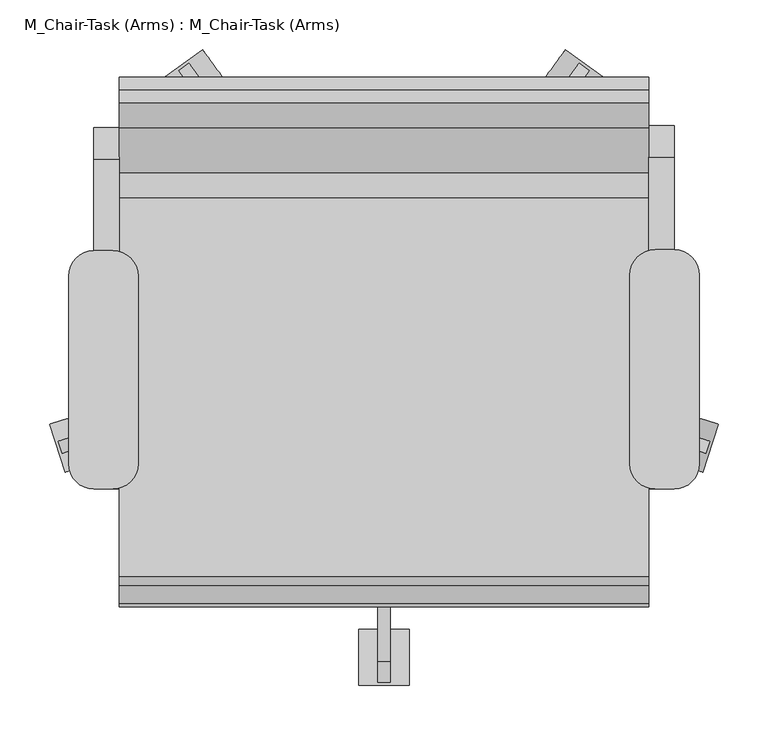
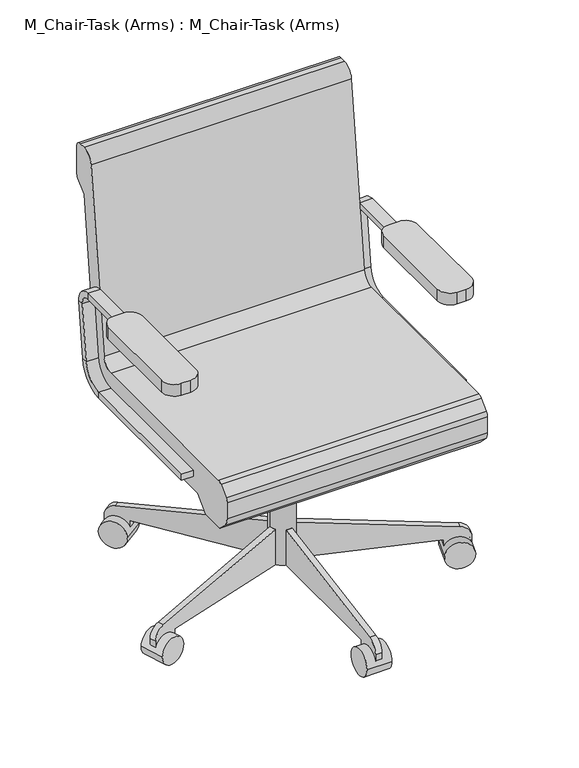
"""IFC4 building model written with IfcOpenShell, lengths in millimetres: furniture geometry, M_Chair-Task (Arms) : M_Chair-Task (Arms)."""

from ifc_helpers import new_model, si_unit, point, frame, frame_2d, origin, place, context, project, spatial, polyline, circle_curve, trimmed, segment, composite_curve, outline, extrude, source, transform, mapped, element, save
from ifc_brep_helpers import plane_surface, cylinder_surface, revolved_surface, advanced_brep


def m_chair_task_arms_m_chair_task_arms_83a3c27c(model_context):
    return source(origin(), model_context, "Body", "SolidModel", [
        extrude(outline(composite_curve([segment(trimmed(circle_curve(frame_2d((126.2050455, 482.6)), 25.4), [point((126.2050455, 457.2))], [point((151.4310708, 479.6322323))], True, "CARTESIAN"), True, "CONTINUOUS"), segment(polyline([(151.4310708, 479.6322323), (196.9528985, 866.5677677)]), True, "CONTINUOUS"), segment(trimmed(circle_curve(frame_2d((222.1789239, 863.6)), 25.4), [point((196.9528985, 866.5677677))], [point((222.1789239, 889.0))], False, "CARTESIAN"), True, "CONTINUOUS"), segment(polyline([(222.1789239, 889.0), (235.0540984, 889.0)]), True, "CONTINUOUS"), segment(trimmed(circle_curve(frame_2d((235.0540984, 876.3)), 12.7), [point((235.0540984, 889.0))], [point((247.7540984, 876.3))], False, "CARTESIAN"), True, "CONTINUOUS"), segment(polyline([(247.7540984, 876.3), (247.7540984, 818.0605122)]), True, "CONTINUOUS"), segment(trimmed(circle_curve(frame_2d((235.0540984, 818.0605122)), 12.7), [point((247.7540984, 818.0605122))], [point((244.0343545, 809.0802561))], False, "CARTESIAN"), True, "CONTINUOUS"), segment(polyline([(244.0343545, 809.0802561), (222.3540984, 787.4), (182.7870738, 451.0802913)]), True, "CONTINUOUS"), segment(trimmed(circle_curve(frame_2d((107.1089978, 459.9835944)), 76.2), [point((182.7870738, 451.0802913))], [point((107.1089978, 383.7835944))], False, "CARTESIAN"), True, "CONTINUOUS"), segment(polyline([(107.1089978, 383.7835944), (-181.0744602, 383.7835944), (-209.4470284, 355.6), (-260.2470284, 355.6), (-278.2663256, 373.7401184)]), True, "CONTINUOUS"), segment(trimmed(circle_curve(frame_2d((-260.2459016, 391.6405184)), 25.4), [point((-278.2663256, 373.7401184))], [point((-285.6459016, 391.6405184))], False, "CARTESIAN"), True, "CONTINUOUS"), segment(polyline([(-285.6459016, 391.6405184), (-285.6459016, 426.6837879)]), True, "CONTINUOUS"), segment(trimmed(circle_curve(frame_2d((-272.9459016, 426.6837879)), 12.7), [point((-285.6459016, 426.6837879))], [point((-281.8961016, 435.6939999))], False, "CARTESIAN"), True, "CONTINUOUS"), segment(polyline([(-281.8961016, 435.6939999), (-263.9604301, 453.510212)]), True, "CONTINUOUS"), segment(trimmed(circle_curve(frame_2d((-255.0102301, 444.5)), 12.7), [point((-263.9604301, 453.510212))], [point((-255.0102301, 457.2))], False, "CARTESIAN"), True, "CONTINUOUS"), segment(polyline([(-255.0102301, 457.2), (126.2050455, 457.2)]), True, "CONTINUOUS")], self_intersect=False)), frame((-125.7091803, 0.0, 0.0), z_axis=(1.0, 0.0, 0.0), x_axis=(0.0, 1.0, 0.0)), (0.0, 0.0, 1.0), 533.4),
        extrude(outline(polyline([(-69.7459016, 383.7835944), (19.1540984, 383.7835944), (19.1540984, 283.0954134), (-18.9459016, 283.0954134), (-69.7459016, 371.0835944), (-69.7459016, 383.7835944)])), frame((90.1908197, 0.0, 0.0), z_axis=(1.0, 0.0, 0.0), x_axis=(0.0, 1.0, 0.0)), (0.0, 0.0, 1.0), 101.6),
        extrude(outline(composite_curve([segment(polyline([(-311.0459016, 53.5835944), (-311.0459016, 28.1835944), (-361.8459016, 28.1835944), (-361.8459016, 52.4866474)]), True, "CONTINUOUS"), segment(trimmed(circle_curve(frame_2d((-336.4459016, 52.4866474)), 25.4), [point((-361.8459016, 52.4866474))], [point((-340.8565654, 77.5007643))], False, "CARTESIAN"), True, "CONTINUOUS"), segment(polyline([(-340.8565654, 77.5007643), (-44.3459016, 129.7835944), (-18.9459016, 129.7835944), (-18.9459016, 53.5835944), (-311.0459016, 53.5835944)]), True, "CONTINUOUS")], self_intersect=False)), frame((134.6408197, 0.0, 0.0), z_axis=(1.0, 0.0, 0.0), x_axis=(0.0, 1.0, 0.0)), (0.0, 0.0, 1.0), 12.7),
        extrude(outline(composite_curve([segment(trimmed(circle_curve(frame_2d((-336.4459016, 28.1835944)), 28.2002727), [point((-308.2456289, 28.1835944))], [point((-364.6461744, 28.1835944))], False, "CARTESIAN"), True, "CONTINUOUS"), segment(trimmed(circle_curve(frame_2d((-336.4459016, 28.1835944)), 28.2002727), [point((-364.6461744, 28.1835944))], [point((-308.2456289, 28.1835944))], False, "CARTESIAN"), True, "CONTINUOUS")], self_intersect=False)), frame((115.5908197, 0.0, 0.0), z_axis=(1.0, 0.0, 0.0), x_axis=(0.0, 1.0, 0.0)), (0.0, 0.0, 1.0), 50.8),
        extrude(outline(composite_curve([segment(polyline([(-25.4, 0.0), (-25.4, -292.1), (-101.6, -292.1), (-101.6, -266.7), (-49.3171699, 29.8106637)]), True, "CONTINUOUS"), segment(trimmed(circle_curve(frame_2d((-24.303053, 25.4)), 25.4), [point((-49.3171699, 29.8106637))], [point((-24.303053, 50.8000001))], False, "CARTESIAN"), True, "CONTINUOUS"), segment(polyline([(-24.303053, 50.8000001), (0.0, 50.8000001), (0.0, 0.0), (-25.4, 0.0)]), True, "CONTINUOUS")], self_intersect=False)), frame((-134.8505308, -115.2489746, 28.1835944), z_axis=(-0.3090169943749487, 0.9510565162951532, 0.0), x_axis=(0.0, 0.0, -1.0)), (0.0, 0.0, 1.0), 12.7),
        extrude(outline(composite_curve([segment(trimmed(circle_curve(frame_2d((0.0, 28.2002727)), 28.2002727), [point((0.0, 56.4005454))], [point((0.0, 0.0))], False, "CARTESIAN"), True, "CONTINUOUS"), segment(trimmed(circle_curve(frame_2d((0.0, 28.2002727)), 28.2002727), [point((0.0, 0.0))], [point((0.0, 56.4005454))], False, "CARTESIAN"), True, "CONTINUOUS")], self_intersect=False)), frame((-179.9406457, -149.9299964, 28.1835944), z_axis=(-0.3090169943749487, 0.9510565162951532, 0.0), x_axis=(0.0, 0.0, 1.0)), (0.0, 0.0, 1.0), 50.8),
        extrude(outline(composite_curve([segment(polyline([(-25.4, 0.0), (-25.4, -292.1), (-101.6, -292.1), (-101.6, -266.6999999), (-49.3171699, 29.8106637)]), True, "CONTINUOUS"), segment(trimmed(circle_curve(frame_2d((-24.303053, 25.3999999)), 25.4), [point((-49.3171699, 29.8106637))], [point((-24.303053, 50.8))], False, "CARTESIAN"), True, "CONTINUOUS"), segment(polyline([(-24.303053, 50.8), (0.0, 50.8), (0.0, 0.0), (-25.4, 0.0)]), True, "CONTINUOUS")], self_intersect=False)), frame((-35.8385104, 213.6355261, 28.1835944), z_axis=(0.8090169943749459, 0.5877852522924754, 0.0), x_axis=(0.0, 0.0, -1.0)), (0.0, 0.0, 1.0), 12.7),
        extrude(outline(composite_curve([segment(trimmed(circle_curve(frame_2d((0.0, 28.2002726)), 28.2002727), [point((0.0, 56.4005454))], [point((0.0, 0.0))], False, "CARTESIAN"), True, "CONTINUOUS"), segment(trimmed(circle_curve(frame_2d((0.0, 28.2002726)), 28.2002727), [point((0.0, 0.0))], [point((0.0, 56.4005454))], False, "CARTESIAN"), True, "CONTINUOUS")], self_intersect=False)), frame((-82.755734, 245.8017485, 28.1835944), z_axis=(0.8090169943749458, 0.5877852522924754, 0.0), x_axis=(0.0, 0.0, 1.0)), (0.0, 0.0, 1.0), 50.8),
        extrude(outline(composite_curve([segment(polyline([(25.4, 0.0), (0.0, 0.0), (0.0, 50.8), (24.303053, 50.8)]), True, "CONTINUOUS"), segment(trimmed(circle_curve(frame_2d((24.303053, 25.3999999)), 25.4), [point((24.303053, 50.8))], [point((49.3171699, 29.8106637))], False, "CARTESIAN"), True, "CONTINUOUS"), segment(polyline([(49.3171699, 29.8106637), (101.6, -266.7), (101.6, -292.1), (25.4, -292.1), (25.4, 0.0)]), True, "CONTINUOUS")], self_intersect=False)), frame((317.8201498, 213.6355261, 28.1835944), z_axis=(-0.8090169943749499, 0.5877852522924699, 0.0), x_axis=(0.0, 0.0, 1.0)), (0.0, 0.0, 1.0), 12.7),
        extrude(outline(composite_curve([segment(trimmed(circle_curve(frame_2d((0.0, 28.2002726)), 28.2002727), [point((0.0, 56.4005454))], [point((0.0, 0.0))], False, "CARTESIAN"), True, "CONTINUOUS"), segment(trimmed(circle_curve(frame_2d((0.0, 28.2002726)), 28.2002727), [point((0.0, 0.0))], [point((0.0, 56.4005454))], False, "CARTESIAN"), True, "CONTINUOUS")], self_intersect=False)), frame((364.7373733, 245.8017485, 28.1835944), z_axis=(-0.8090169943749499, 0.5877852522924699, 0.0), x_axis=(0.0, 0.0, -1.0)), (0.0, 0.0, 1.0), 50.8),
        extrude(outline(composite_curve([segment(polyline([(25.4, 0.0), (0.0, 0.0), (0.0, 50.8), (24.303053, 50.8)]), True, "CONTINUOUS"), segment(trimmed(circle_curve(frame_2d((24.303053, 25.4)), 25.4), [point((24.303053, 50.8))], [point((49.3171699, 29.8106636))], False, "CARTESIAN"), True, "CONTINUOUS"), segment(polyline([(49.3171699, 29.8106636), (101.6, -266.7), (101.6, -292.1), (25.4, -292.1), (25.4, 0.0)]), True, "CONTINUOUS")], self_intersect=False)), frame((416.8321702, -115.2489746, 28.1835944), z_axis=(0.3090169943749423, 0.9510565162951553, 0.0), x_axis=(0.0, 0.0, 1.0)), (0.0, 0.0, 1.0), 12.7),
        extrude(outline(composite_curve([segment(trimmed(circle_curve(frame_2d((0.0, 28.2002728)), 28.2002727), [point((0.0, 56.4005455))], [point((0.0, 0.0))], False, "CARTESIAN"), True, "CONTINUOUS"), segment(trimmed(circle_curve(frame_2d((0.0, 28.2002728)), 28.2002727), [point((0.0, 0.0))], [point((0.0, 56.4005455))], False, "CARTESIAN"), True, "CONTINUOUS")], self_intersect=False)), frame((461.9222851, -149.9299964, 28.1835944), z_axis=(0.3090169943749423, 0.9510565162951553, 0.0), x_axis=(0.0, 0.0, -1.0)), (0.0, 0.0, 1.0), 50.8),
        extrude(outline(composite_curve([segment(trimmed(circle_curve(frame_2d((140.9908197, -18.9459016)), 25.4), [point((115.5908197, -18.9459016))], [point((166.3908197, -18.9459016))], False, "CARTESIAN"), True, "CONTINUOUS"), segment(trimmed(circle_curve(frame_2d((140.9908197, -18.9459016)), 25.4), [point((166.3908197, -18.9459016))], [point((115.5908197, -18.9459016))], False, "CARTESIAN"), True, "CONTINUOUS")], self_intersect=False)), frame((0.0, 0.0, 53.5835944), z_axis=(0.0, 0.0, 1.0), x_axis=(1.0, 0.0, 0.0)), (0.0, 0.0, 1.0), 330.5914056),
        advanced_brep(
        [(433.0908197, -167.0319091, 425.45), (407.6908197, -167.0319091, 425.45), (407.6908197, -167.0319091, 412.75), (433.0908197, -167.0319091, 412.75), (433.0908197, 128.329278, 412.75), (433.0908197, 128.329278, 425.45), (407.6908197, 128.329278, 412.75), (407.6908197, 128.329278, 425.45), (433.0908197, 185.0878351, 463.2225227), (433.0908197, 172.4748224, 464.7064065), (407.6908197, 185.0878351, 463.2225227), (407.6908197, 172.4748224, 464.7064065), (433.0908197, 198.884043, 580.4902904), (433.0908197, 186.2710303, 581.9741742), (407.6908197, 198.884043, 580.4902904), (407.6908197, 186.2710303, 581.9741742), (433.0908197, 167.3515113, 615.95), (433.0908197, 167.3515113, 603.25), (407.6908197, 167.3515113, 615.95), (407.6908197, 167.3515113, 603.25), (433.0908197, -18.9459016, 603.25), (433.0908197, -18.9459016, 615.95), (407.6908197, -18.9459016, 615.95), (407.6908197, -18.9459016, 603.25)],
        [
            (0, 1),
            (1, 2),
            (2, 3),
            (3, 0),
            (3, 4),
            (4, 5),
            (5, 0),
            (2, 6),
            (6, 4),
            (1, 7),
            (7, 6),
            (5, 7),
            (8, 9),
            (9, 5, circle_curve(frame((433.0908197, 128.329278, 469.9), z_axis=(-1.0, 0.0, 0.0), x_axis=(0.0, 0.0, -1.0)), 44.45)),
            (4, 8, circle_curve(frame((433.0908197, 128.329278, 469.9), z_axis=(1.0, 0.0, 0.0), x_axis=(0.0, 0.0, -1.0)), 57.15)),
            (10, 8),
            (6, 10, circle_curve(frame((407.6908197, 128.329278, 469.9), z_axis=(1.0, 0.0, 0.0), x_axis=(0.0, 0.0, -1.0)), 57.15)),
            (11, 10),
            (7, 11, circle_curve(frame((407.6908197, 128.329278, 469.9), z_axis=(1.0, 0.0, 0.0), x_axis=(0.0, 0.0, -1.0)), 44.45)),
            (9, 11),
            (8, 12),
            (12, 13),
            (13, 9),
            (10, 14),
            (14, 12),
            (11, 15),
            (15, 14),
            (13, 15),
            (16, 17),
            (17, 13, circle_curve(frame((433.0908197, 167.3515113, 584.2), z_axis=(-1.0, 0.0, 0.0), x_axis=(0.0, 0.9931506043228767, -0.1168412475673929)), 19.05)),
            (12, 16, circle_curve(frame((433.0908197, 167.3515113, 584.2), z_axis=(1.0, 0.0, 0.0), x_axis=(0.0, 0.9931506043228767, -0.1168412475673929)), 31.75)),
            (18, 16),
            (14, 18, circle_curve(frame((407.6908197, 167.3515113, 584.2), z_axis=(1.0, 0.0, 0.0), x_axis=(0.0, 0.9931506043228767, -0.1168412475673929)), 31.75)),
            (19, 18),
            (15, 19, circle_curve(frame((407.6908197, 167.3515113, 584.2), z_axis=(1.0, 0.0, 0.0), x_axis=(0.0, 0.9931506043228767, -0.1168412475673929)), 19.05)),
            (17, 19),
            (20, 21),
            (21, 22),
            (22, 23),
            (23, 20),
            (16, 21),
            (20, 17),
            (18, 22),
            (19, 23),
        ],
        [
            plane_surface(frame((406.191788, -167.0319091, 419.1), z_axis=(0.0, -1.0, 0.0), x_axis=(0.0, 0.0, -1.0))),
            plane_surface(frame((433.0908197, -167.0319091, 425.45), z_axis=(1.0, 0.0, 0.0), x_axis=(0.0, 1.0, 0.0))),
            plane_surface(frame((433.0908197, -167.0319091, 412.75), z_axis=(0.0, 0.0, -1.0), x_axis=(0.0, 1.0, 0.0))),
            plane_surface(frame((407.6908197, -167.0319091, 412.75), z_axis=(-1.0, 0.0, 0.0), x_axis=(0.0, 1.0, 0.0))),
            plane_surface(frame((407.6908197, -167.0319091, 425.45), z_axis=(0.0, 0.0, 1.0), x_axis=(0.0, 1.0, 0.0))),
            plane_surface(frame((433.0908197, 128.329278, 469.9), z_axis=(1.0, 0.0, 0.0), x_axis=(0.0, 0.0, -1.0))),
            cylinder_surface(frame((420.3908197, 128.329278, 469.9), z_axis=(-1.0, 0.0, 0.0), x_axis=(0.0, 0.0, -1.0)), 57.15),
            plane_surface(frame((407.6908197, 128.329278, 469.9), z_axis=(-1.0, 0.0, 0.0), x_axis=(0.0, 0.0, -1.0))),
            revolved_surface(polyline([(407.6908197, 128.329278, 425.45), (433.0908197, 128.329278, 425.45)]), (420.3908197, 128.329278, 469.9), (-1.0, 0.0, 0.0)),
            plane_surface(frame((433.0908197, 172.4748224, 464.7064065), z_axis=(1.0, 0.0, 0.0), x_axis=(0.0, 0.11684124756738626, 0.9931506043228775))),
            plane_surface(frame((433.0908197, 185.0878351, 463.2225227), z_axis=(0.0, 0.9931506043228775, -0.11684124756738655), x_axis=(0.0, 0.11684124756738655, 0.9931506043228775))),
            plane_surface(frame((407.6908197, 185.0878351, 463.2225227), z_axis=(-1.0, 0.0, 0.0), x_axis=(0.0, 0.11684124756738626, 0.9931506043228775))),
            plane_surface(frame((407.6908197, 172.4748224, 464.7064065), z_axis=(0.0, -0.9931506043228775, 0.11684124756738626), x_axis=(0.0, 0.11684124756738626, 0.9931506043228775))),
            plane_surface(frame((433.0908197, 167.3515113, 584.2), z_axis=(1.0, 0.0, 0.0), x_axis=(0.0, 0.9931506043228767, -0.1168412475673929))),
            cylinder_surface(frame((420.3908197, 167.3515113, 584.2), z_axis=(-1.0, 0.0, 0.0), x_axis=(0.0, 0.9931506043228767, -0.1168412475673929)), 31.75),
            plane_surface(frame((407.6908197, 167.3515113, 584.2), z_axis=(-1.0, 0.0, 0.0), x_axis=(0.0, 0.9931506043228767, -0.1168412475673929))),
            revolved_surface(polyline([(407.6908197, 186.2710303123508, 581.9741742338412), (433.0908197, 186.2710303123508, 581.9741742338412)]), (420.3908197, 167.3515113, 584.2), (-1.0, 0.0, 0.0)),
            plane_surface(frame((406.191788, -18.9459016, 609.6), z_axis=(0.0, -1.0, 0.0), x_axis=(0.0, 0.0, 1.0))),
            plane_surface(frame((433.0908197, 167.3515113, 603.25), z_axis=(1.0, 0.0, 0.0), x_axis=(0.0, -1.0, 0.0))),
            plane_surface(frame((433.0908197, 167.3515113, 615.95), z_axis=(0.0, 0.0, 1.0), x_axis=(0.0, -1.0, 0.0))),
            plane_surface(frame((407.6908197, 167.3515113, 615.95), z_axis=(-1.0, 0.0, 0.0), x_axis=(0.0, -1.0, 0.0))),
            plane_surface(frame((407.6908197, 167.3515113, 603.25), z_axis=(0.0, 0.0, -1.0), x_axis=(0.0, -1.0, 0.0))),
        ],
        [
            (0, [[1, 2, 3, 4]]),
            (1, [[5, 6, 7, -4]]),
            (2, [[8, 9, -5, -3]]),
            (3, [[10, 11, -8, -2]]),
            (4, [[-7, 12, -10, -1]]),
            (5, [[13, 14, -6, 15]]),
            (6, [[16, -15, -9, 17]]),
            (7, [[18, -17, -11, 19]]),
            (8, [[20, -19, -12, -14]]),
            (9, [[21, 22, 23, -13]]),
            (10, [[24, 25, -21, -16]]),
            (11, [[26, 27, -24, -18]]),
            (12, [[-23, 28, -26, -20]]),
            (13, [[29, 30, -22, 31]]),
            (14, [[32, -31, -25, 33]]),
            (15, [[34, -33, -27, 35]]),
            (16, [[36, -35, -28, -30]]),
            (17, [[37, 38, 39, 40]]),
            (18, [[41, -37, 42, -29]]),
            (19, [[43, -38, -41, -32]]),
            (20, [[44, -39, -43, -34]]),
            (21, [[-42, -40, -44, -36]]),
        ],
    ),
        advanced_brep(
        [(-151.1091803, -167.0319091, 412.75), (-125.7091803, -167.0319091, 412.75), (-125.7091803, -167.0319091, 425.45), (-151.1091803, -167.0319091, 425.45), (-151.1091803, 126.2388651, 425.45), (-151.1091803, 126.2388651, 412.75), (-125.7091803, 126.2388651, 425.45), (-125.7091803, 126.2388651, 412.75), (-151.1091803, 170.3844094, 464.7064065), (-151.1091803, 182.9974221, 463.2225227), (-125.7091803, 170.3844094, 464.7064065), (-125.7091803, 182.9974221, 463.2225227), (-151.1091803, 184.1806174, 581.9741742), (-151.1091803, 196.7936301, 580.4902904), (-125.7091803, 184.1806174, 581.9741742), (-125.7091803, 196.7936301, 580.4902904), (-151.1091803, 165.2610984, 603.25), (-151.1091803, 165.2610984, 615.95), (-125.7091803, 165.2610984, 603.25), (-125.7091803, 165.2610984, 615.95), (-151.1091803, -18.9459016, 615.95), (-151.1091803, -18.9459016, 603.25), (-125.7091803, -18.9459016, 603.25), (-125.7091803, -18.9459016, 615.95)],
        [
            (0, 1),
            (1, 2),
            (2, 3),
            (3, 0),
            (3, 4),
            (4, 5),
            (5, 0),
            (2, 6),
            (6, 4),
            (1, 7),
            (7, 6),
            (5, 7),
            (8, 9),
            (9, 5, circle_curve(frame((-151.1091803, 126.2388651, 469.9), z_axis=(-1.0, 0.0, 0.0), x_axis=(0.0, 0.0, -1.0)), 57.15)),
            (4, 8, circle_curve(frame((-151.1091803, 126.2388651, 469.9), z_axis=(1.0, 0.0, 0.0), x_axis=(0.0, 0.0, -1.0)), 44.45)),
            (10, 8),
            (6, 10, circle_curve(frame((-125.7091803, 126.2388651, 469.9), z_axis=(1.0, 0.0, 0.0), x_axis=(0.0, 0.0, -1.0)), 44.45)),
            (11, 10),
            (7, 11, circle_curve(frame((-125.7091803, 126.2388651, 469.9), z_axis=(1.0, 0.0, 0.0), x_axis=(0.0, 0.0, -1.0)), 57.15)),
            (9, 11),
            (8, 12),
            (12, 13),
            (13, 9),
            (10, 14),
            (14, 12),
            (11, 15),
            (15, 14),
            (13, 15),
            (16, 17),
            (17, 13, circle_curve(frame((-151.1091803, 165.2610984, 584.2), z_axis=(-1.0, 0.0, 0.0), x_axis=(0.0, 0.9931506043228768, -0.11684124756739202)), 31.75)),
            (12, 16, circle_curve(frame((-151.1091803, 165.2610984, 584.2), z_axis=(1.0, 0.0, 0.0), x_axis=(0.0, 0.9931506043228768, -0.11684124756739202)), 19.05)),
            (18, 16),
            (14, 18, circle_curve(frame((-125.7091803, 165.2610984, 584.2), z_axis=(1.0, 0.0, 0.0), x_axis=(0.0, 0.9931506043228768, -0.11684124756739202)), 19.05)),
            (19, 18),
            (15, 19, circle_curve(frame((-125.7091803, 165.2610984, 584.2), z_axis=(1.0, 0.0, 0.0), x_axis=(0.0, 0.9931506043228768, -0.11684124756739202)), 31.75)),
            (17, 19),
            (20, 21),
            (21, 22),
            (22, 23),
            (23, 20),
            (16, 21),
            (20, 17),
            (18, 22),
            (19, 23),
        ],
        [
            plane_surface(frame((-152.608212, -167.0319091, 419.1), z_axis=(0.0, -1.0, 0.0), x_axis=(0.0, 0.0, -1.0))),
            plane_surface(frame((-151.1091803, -167.0319091, 412.75), z_axis=(-1.0, 0.0, 0.0), x_axis=(0.0, 1.0, 0.0))),
            plane_surface(frame((-151.1091803, -167.0319091, 425.45), z_axis=(0.0, 0.0, 1.0), x_axis=(0.0, 1.0, 0.0))),
            plane_surface(frame((-125.7091803, -167.0319091, 425.45), z_axis=(1.0, 0.0, 0.0), x_axis=(0.0, 1.0, 0.0))),
            plane_surface(frame((-125.7091803, -167.0319091, 412.75), z_axis=(0.0, 0.0, -1.0), x_axis=(0.0, 1.0, 0.0))),
            plane_surface(frame((-151.1091803, 126.2388651, 469.9), z_axis=(-1.0, 0.0, 0.0), x_axis=(0.0, 0.0, -1.0))),
            revolved_surface(polyline([(-151.1091803, 126.2388651, 425.45), (-125.7091803, 126.2388651, 425.45)]), (-138.4091803, 126.2388651, 469.9), (-1.0, 0.0, 0.0)),
            plane_surface(frame((-125.7091803, 126.2388651, 469.9), z_axis=(1.0, 0.0, 0.0), x_axis=(0.0, 0.0, -1.0))),
            cylinder_surface(frame((-138.4091803, 126.2388651, 469.9), z_axis=(-1.0, 0.0, 0.0), x_axis=(0.0, 0.0, -1.0)), 57.15),
            plane_surface(frame((-151.1091803, 182.9974221, 463.2225227), z_axis=(-1.0, 0.0, 0.0), x_axis=(0.0, 0.1168412475673856, 0.9931506043228776))),
            plane_surface(frame((-151.1091803, 170.3844094, 464.7064065), z_axis=(0.0, -0.9931506043228776, 0.1168412475673856), x_axis=(0.0, 0.1168412475673856, 0.9931506043228776))),
            plane_surface(frame((-125.7091803, 170.3844094, 464.7064065), z_axis=(1.0, 0.0, 0.0), x_axis=(0.0, 0.1168412475673856, 0.9931506043228776))),
            plane_surface(frame((-125.7091803, 182.9974221, 463.2225227), z_axis=(0.0, 0.9931506043228776, -0.1168412475673856), x_axis=(0.0, 0.1168412475673856, 0.9931506043228776))),
            plane_surface(frame((-151.1091803, 165.2610984, 584.2), z_axis=(-1.0, 0.0, 0.0), x_axis=(0.0, 0.9931506043228768, -0.11684124756739202))),
            revolved_surface(polyline([(-151.1091803, 184.1806174123508, 581.9741742338413), (-125.7091803, 184.1806174123508, 581.9741742338413)]), (-138.4091803, 165.2610984, 584.2), (-1.0, 0.0, 0.0)),
            plane_surface(frame((-125.7091803, 165.2610984, 584.2), z_axis=(1.0, 0.0, 0.0), x_axis=(0.0, 0.9931506043228768, -0.11684124756739202))),
            cylinder_surface(frame((-138.4091803, 165.2610984, 584.2), z_axis=(-1.0, 0.0, 0.0), x_axis=(0.0, 0.9931506043228768, -0.11684124756739202)), 31.75),
            plane_surface(frame((-152.608212, -18.9459016, 609.6), z_axis=(0.0, -1.0, 0.0), x_axis=(0.0, 0.0, 1.0))),
            plane_surface(frame((-151.1091803, 165.2610984, 615.95), z_axis=(-1.0, 0.0, 0.0), x_axis=(0.0, -1.0, 0.0))),
            plane_surface(frame((-151.1091803, 165.2610984, 603.25), z_axis=(0.0, 0.0, -1.0), x_axis=(0.0, -1.0, 0.0))),
            plane_surface(frame((-125.7091803, 165.2610984, 603.25), z_axis=(1.0, 0.0, 0.0), x_axis=(0.0, -1.0, 0.0))),
            plane_surface(frame((-125.7091803, 165.2610984, 615.95), z_axis=(0.0, 0.0, 1.0), x_axis=(0.0, -1.0, 0.0))),
        ],
        [
            (0, [[1, 2, 3, 4]]),
            (1, [[5, 6, 7, -4]]),
            (2, [[8, 9, -5, -3]]),
            (3, [[10, 11, -8, -2]]),
            (4, [[-7, 12, -10, -1]]),
            (5, [[13, 14, -6, 15]]),
            (6, [[16, -15, -9, 17]]),
            (7, [[18, -17, -11, 19]]),
            (8, [[20, -19, -12, -14]]),
            (9, [[21, 22, 23, -13]]),
            (10, [[24, 25, -21, -16]]),
            (11, [[26, 27, -24, -18]]),
            (12, [[-23, 28, -26, -20]]),
            (13, [[29, 30, -22, 31]]),
            (14, [[32, -31, -25, 33]]),
            (15, [[34, -33, -27, 35]]),
            (16, [[36, -35, -28, -30]]),
            (17, [[37, 38, 39, 40]]),
            (18, [[41, -37, 42, -29]]),
            (19, [[43, -38, -41, -32]]),
            (20, [[44, -39, -43, -34]]),
            (21, [[-42, -40, -44, -36]]),
        ],
    ),
        extrude(outline(composite_curve([segment(trimmed(circle_curve(frame_2d((433.0908197, 48.8028048)), 25.4), [point((433.0908197, 74.2028048))], [point((458.4908197, 48.8028048))], False, "CARTESIAN"), True, "CONTINUOUS"), segment(polyline([(458.4908197, 48.8028048), (458.4908197, -141.6319091)]), True, "CONTINUOUS"), segment(trimmed(circle_curve(frame_2d((433.0908197, -141.6319091)), 25.4), [point((458.4908197, -141.6319091))], [point((433.0908197, -167.0319091))], False, "CARTESIAN"), True, "CONTINUOUS"), segment(polyline([(433.0908197, -167.0319091), (414.0408197, -167.0319091)]), True, "CONTINUOUS"), segment(trimmed(circle_curve(frame_2d((414.0408197, -141.6319091)), 25.4), [point((414.0408197, -167.0319091))], [point((388.6408197, -141.6319091))], False, "CARTESIAN"), True, "CONTINUOUS"), segment(polyline([(388.6408197, -141.6319091), (388.6408197, 48.8028048)]), True, "CONTINUOUS"), segment(trimmed(circle_curve(frame_2d((414.0408197, 48.8028048)), 25.4), [point((388.6408197, 48.8028048))], [point((414.0408197, 74.2028048))], False, "CARTESIAN"), True, "CONTINUOUS"), segment(polyline([(414.0408197, 74.2028048), (433.0908197, 74.2028048)]), True, "CONTINUOUS")], self_intersect=False)), frame((0.0, 0.0, 596.9), z_axis=(0.0, 0.0, 1.0), x_axis=(1.0, 0.0, 0.0)), (0.0, 0.0, 1.0), 25.4),
        extrude(outline(composite_curve([segment(trimmed(circle_curve(frame_2d((-132.0591803, 47.7575984)), 25.4), [point((-132.0591803, 73.1575984))], [point((-106.6591803, 47.7575984))], False, "CARTESIAN"), True, "CONTINUOUS"), segment(polyline([(-106.6591803, 47.7575984), (-106.6591803, -141.6319091)]), True, "CONTINUOUS"), segment(trimmed(circle_curve(frame_2d((-132.0591803, -141.6319091)), 25.4), [point((-106.6591803, -141.6319091))], [point((-132.0591803, -167.0319091))], False, "CARTESIAN"), True, "CONTINUOUS"), segment(polyline([(-132.0591803, -167.0319091), (-151.1091803, -167.0319091)]), True, "CONTINUOUS"), segment(trimmed(circle_curve(frame_2d((-151.1091803, -141.6319091)), 25.4), [point((-151.1091803, -167.0319091))], [point((-176.5091803, -141.6319091))], False, "CARTESIAN"), True, "CONTINUOUS"), segment(polyline([(-176.5091803, -141.6319091), (-176.5091803, 47.7575984)]), True, "CONTINUOUS"), segment(trimmed(circle_curve(frame_2d((-151.1091803, 47.7575984)), 25.4), [point((-176.5091803, 47.7575984))], [point((-151.1091803, 73.1575984))], False, "CARTESIAN"), True, "CONTINUOUS"), segment(polyline([(-151.1091803, 73.1575984), (-132.0591803, 73.1575984)]), True, "CONTINUOUS")], self_intersect=False)), frame((0.0, 0.0, 596.9), z_axis=(0.0, 0.0, 1.0), x_axis=(1.0, 0.0, 0.0)), (0.0, 0.0, 1.0), 25.4),
    ])


if __name__ == "__main__":
    model = new_model("IFC4")
    model_context = context("Model", 3, world=origin())
    ifc_project = project(units=[si_unit("LENGTHUNIT", "METRE", prefix="MILLI")], contexts=[model_context])
    site = spatial("IfcSite", under=ifc_project)
    building = spatial("IfcBuilding", under=site)
    placement = place(None, origin())
    m_chair_task_arms_m_chair_task_arms_shape = m_chair_task_arms_m_chair_task_arms_83a3c27c(model_context)
    element("IfcFurniture", 1, ObjectType="M_Chair-Task (Arms) : M_Chair-Task (Arms)", at=placement, inside=building, context=model_context, shape_type="MappedRepresentation", body=[
        mapped(m_chair_task_arms_m_chair_task_arms_shape, transform((0.0, 0.0, 0.0), x_axis=(1.0, 0.0, 0.0), y_axis=(0.0, 1.0, 0.0), z_axis=(0.0, 0.0, 1.0))),
    ])
    save(model, "model.ifc")

# Revit data of these elements
# Type "M_Chair-Task (Arms) : M_Chair-Task (Arms)"
#   Base Material = Plastic, Opaque Black
#   Caster Material = Plastic, Opaque Black
#   Seat/Back Material = Textile - Slate Blue
#   Default Elevation = 0
# Element 1 (IfcFurniture, "M_Chair-Task (Arms) : M_Chair-Task (Arms)")
#   Materials on its faces: "Plastic, Opaque Black", "Textile - Slate Blue"
# Materials
#   "Plastic, Opaque Black": class "Plastic", colour RGB 0 0 0, transparency 0.7, Description = "Plastic, generic, opaque black", Cost = 0
#   "Textile - Slate Blue": class "Fabric", colour RGB 98 102 118, transparency 0
